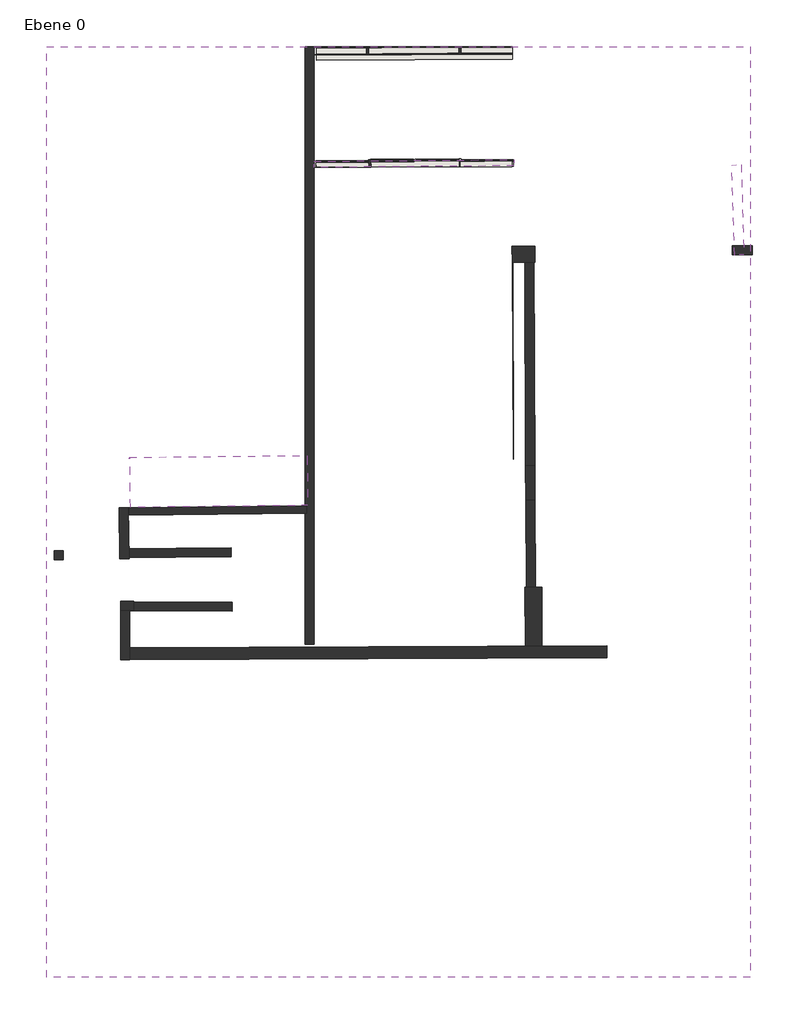
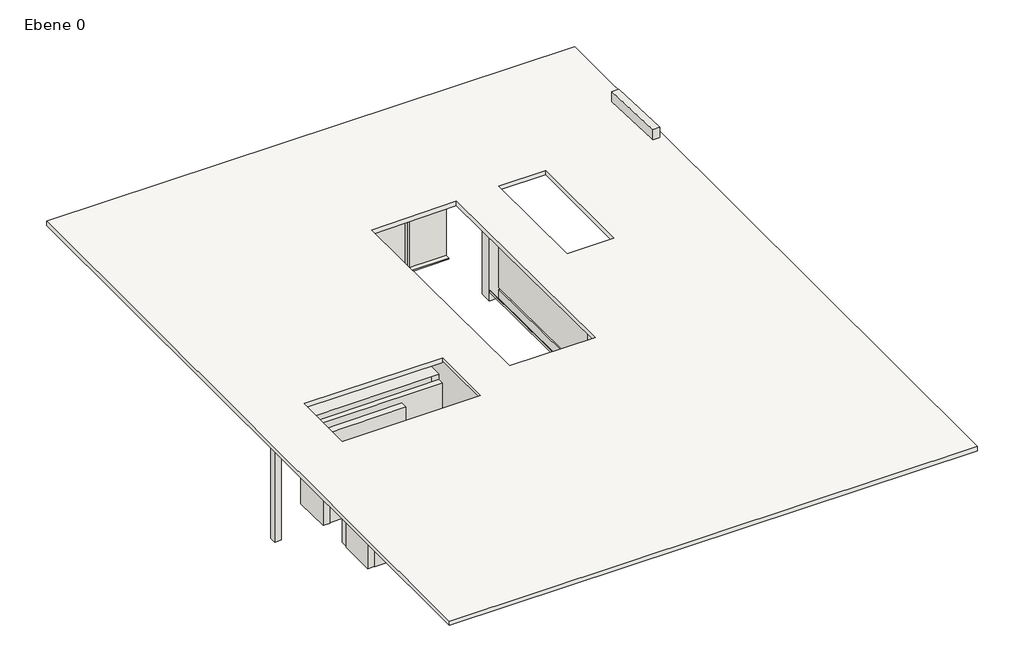
# One storey: 46 walls, 1 slab.
"""IFC4 building model written with IfcOpenShell, lengths in millimetres."""

from ifc_helpers import new_model, si_unit, frame, origin, place, context, project, spatial, polyline, outline, extrude, faceted_brep, element, save

model = new_model("IFC4")

# Units and contexts
model_context = context("Model", 3, world=origin())
ifc_project = project(units=[si_unit("LENGTHUNIT", "METRE", prefix="MILLI")], contexts=[model_context])

# Site, building, storey
site = spatial("IfcSite", under=ifc_project)
building = spatial("IfcBuilding", under=site)
storey = spatial("IfcBuildingStorey", under=building, Name="Ebene 0", Elevation=0.0)

# Slab
placement = place(None, origin())
element("IfcSlab", 1, ObjectType="STB 20.0", at=placement, inside=storey, context=model_context, shape_type="SweptSolid", body=[
    extrude(outline(polyline([(-11157.8712691, 14929.5123719), (12093.7927353, 14929.5123719), (12093.7927353, -15793.3401329), (-11157.8712691, -15793.3401329), (-11157.8712691, 14929.5123719)]), holes=[polyline([(-714.2464416, 8224.8662101), (-668.7269694, -2221.6847127), (3095.1356268, -2221.8899612), (3040.6752554, 8277.9612695), (-714.2464416, 8224.8662101)]), polyline([(4959.6247998, 8341.5505497), (4959.6247998, 3140.1225236), (7016.8801574, 3140.1225236), (7016.8801574, 8341.5505497), (4959.6247998, 8341.5505497)]), polyline([(-2623.9258692, -3380.2933626), (-2623.9258692, -499.2133132), (-8707.8712691, -499.2133132), (-8707.8712691, -3380.2933626), (-2623.9258692, -3380.2933626)])]), frame((0.0, 0.0, 3005.0), z_axis=(0.0, 0.0, 1.0), x_axis=(1.0, 0.0, 0.0)), (0.0, 0.0, 1.0), 200.0),
])

# Walls
element("IfcWall", 2, ObjectType="STB 30.0 - Sichtbeton 1", at=placement, inside=storey, context=model_context, shape_type="SweptSolid", body=[
    extrude(outline(polyline([(-8402.8984862, -3386.1116182), (-5023.0576004, -3407.986993), (-5024.9992525, -3707.9807096), (-8404.8401383, -3686.1053348), (-8402.8984862, -3386.1116182)])), frame((0.0, 0.0, -1567.0079424), z_axis=(0.0, 0.0, 1.0), x_axis=(1.0, 0.0, 0.0)), (0.0, 0.0, 1.0), 4193.9637451),
])
element("IfcWall", 3, ObjectType="STB 30.0 - Sichtbeton 1", at=placement, inside=storey, context=model_context, shape_type="SweptSolid", body=[
    extrude(outline(polyline([(-8711.881099, -1641.309095), (-5062.179794, -1608.676683), (-5059.4975656, -1908.6646922), (-8709.1988706, -1941.2971042), (-8711.881099, -1641.309095)])), frame((0.0, 0.0, -1566.6113359), z_axis=(0.0, 0.0, 1.0), x_axis=(1.0, 0.0, 0.0)), (0.0, 0.0, 1.0), 4193.494873),
])
element("IfcWall", 4, ObjectType="STB 30.0 - Sichtbeton 1", at=placement, inside=storey, context=model_context, shape_type="Brep", body=[
    faceted_brep([(-8280.7224922, -3375.8727385, -1505.4189133), (-8707.8712691, -3380.2933626, -1505.4189133), (-8707.8712691, -3380.2933626, 2636.550325), (-8280.7224922, -3375.8727385, 2636.550325), (-8280.7224922, -3375.8727385, -1388.9973215), (-8280.4523049, -3675.8860076, -1505.4189133), (-8280.4523049, -3675.8860076, 2636.550325), (-8407.8712691, -3677.2046848, 2636.550325), (-8707.8712691, -3680.3094278, 2636.550325), (-8707.8712691, -3680.3094278, -1505.4189133)], [[[0, 1, 2, 3, 4]], [[5, 6, 7, 8, 9]], [[1, 0, 5, 9]], [[3, 2, 8, 7, 6]], [[0, 4, 3, 6, 5]], [[2, 1, 9, 8]]]),
])
element("IfcWall", 5, ObjectType="STB 30.0 - Sichtbeton 1", at=placement, inside=storey, context=model_context, shape_type="Brep", body=[
    faceted_brep([(-8407.8712691, -5310.6242916, -1565.0), (-8407.8712691, -3677.2046848, -1565.0), (-8407.8712691, -3677.2046848, 2636.550325), (-8407.8712691, -5310.6242916, 2636.550325), (-8707.8712691, -5312.0476748, -1565.0), (-8707.8712691, -5312.0476748, 2636.550325), (-8707.8712691, -3680.3094278, 2636.550325), (-8707.8712691, -3680.3094278, -1505.4189133), (-8707.8712691, -3680.3094278, -1565.0)], [[[0, 1, 2, 3]], [[4, 5, 6, 7, 8]], [[1, 0, 4, 8]], [[3, 2, 6, 5]], [[2, 1, 8, 7, 6]], [[0, 3, 5, 4]]]),
])
element("IfcWall", 6, ObjectType="STB 30.0 - Sichtbeton 1", at=placement, inside=storey, context=model_context, shape_type="SweptSolid", body=[
    extrude(outline(polyline([(-8454.8872938, -283.8713377), (-8435.0535607, -1969.7388339), (-8735.0328016, -1973.268001), (-8754.8665347, -287.4005048), (-8454.8872938, -283.8713377)])), frame((0.0, 0.0, -1567.5369553), z_axis=(0.0, 0.0, 1.0), x_axis=(1.0, 0.0, 0.0)), (0.0, 0.0, 1.0), 4195.9727783),
])
element("IfcWall", 7, ObjectType="STB 30.0 - Sichtbeton 1", at=placement, inside=storey, context=model_context, shape_type="SweptSolid", body=[
    extrude(outline(polyline([(-10898.8481887, -2010.6735209), (-10902.7495019, -1710.7000992), (-10602.7748702, -1706.7987702), (-10598.873557, -2006.772192), (-10898.8481887, -2010.6735209)])), frame((0.0, 0.0, -1564.2386155), z_axis=(0.0, 0.0, 1.0), x_axis=(1.0, 0.0, 0.0)), (0.0, 0.0, 1.0), 4321.9161377),
])
element("IfcWall", 8, ObjectType="STB 30.0 - Sichtbeton 1", at=placement, inside=storey, context=model_context, shape_type="Brep", body=[
    faceted_brep([(4640.0905057, 7800.3536755, -1082.1717735), (4667.2831216, 1312.227188, -1082.1717735), (4667.2831216, 1312.227188, -1172.1717735), (4640.0905057, 7800.3536755, -1172.1717735), (4640.0905057, 7800.3536755, -1570.8115996), (4668.150891, 1105.1784267, -1570.8115996), (4668.150891, 1105.1784267, 3029.0079909), (4640.0905057, 7800.3536755, 3029.0079909), (4940.0878709, 7801.6110051, -1082.1717735), (4940.0878709, 7801.6110051, 3029.0079909), (4968.1456336, 1107.0614957, 3029.0079909), (4968.1456336, 1107.0614957, -1570.8115996), (4940.0878709, 7801.6110051, -1570.8115996), (4940.0878709, 7801.6110051, -1172.1717735), (4967.2804868, 1313.4845175, -1172.1717735), (4967.2804868, 1313.4845175, -1082.1717735)], [[[0, 1, 2, 3, 4, 5, 6, 7]], [[8, 9, 10, 11, 12, 13, 14, 15]], [[1, 0, 8, 15]], [[2, 1, 15, 14]], [[3, 2, 14, 13]], [[4, 3, 13, 12]], [[5, 4, 12, 11]], [[7, 6, 10, 9]], [[0, 7, 9, 8]], [[6, 5, 11, 10]]]),
])
element("IfcWall", 9, ObjectType="STB 30.0 - Sichtbeton 1", at=placement, inside=storey, context=model_context, shape_type="Brep", body=[
    faceted_brep([(4677.6567247, -31.4843616, 3026.055442), (4668.150891, 1105.1784267, 3026.055442), (4668.150891, 1105.1784267, 833.3), (4668.1769602, 1102.061196, 833.3), (4668.1769602, 1102.061196, 843.3), (4677.6567247, -31.4843616, 843.3), (4968.1456336, 1107.0614956, 3026.055442), (4977.6502256, -29.4528133, 3026.055442), (4977.6502256, -29.4528133, 843.3), (4968.1664699, 1104.5699879, 843.3), (4968.1664699, 1104.5699879, 833.3), (4968.1456336, 1107.0614956, 833.3)], [[[0, 1, 2, 3, 4, 5]], [[6, 7, 8, 9, 10, 11]], [[2, 11, 10, 3]], [[1, 0, 7, 6]], [[2, 1, 6, 11]], [[7, 0, 5, 8]], [[4, 9, 8, 5]], [[9, 4, 3, 10]]]),
])
element("IfcWall", 10, ObjectType="STB 30.0 - Sichtbeton 1", at=placement, inside=storey, context=model_context, shape_type="Brep", body=[
    faceted_brep([(4692.6152809, -2918.6509775, 3026.055442), (4677.6567247, -31.4843616, 3026.055442), (4677.6567247, -31.4843616, 843.3), (4677.6567247, -31.4843616, -1570.8115996), (4677.6744168, -34.8991368, -1570.8115996), (4692.6152809, -2918.6509775, -1570.8115996), (4992.6112545, -2917.0966832, 3026.055442), (4992.6112545, -2917.0966832, -1570.8115996), (4977.665445, -32.3903322, -1570.8115996), (4977.6502256, -29.4528134, -1570.8115996), (4977.6502256, -29.4528134, 843.3), (4977.6502256, -29.4528134, 3026.055442)], [[[0, 1, 2, 3, 4, 5]], [[6, 7, 8, 9, 10, 11]], [[1, 0, 6, 11]], [[5, 4, 3, 9, 8, 7]], [[0, 5, 7, 6]], [[3, 2, 1, 11, 10, 9]]]),
])
element("IfcWall", 11, ObjectType="STB 30.0 - Sichtbeton 1", at=placement, inside=storey, context=model_context, shape_type="Brep", body=[
    faceted_brep([(-2623.9258692, -4796.8405571, -1559.2743428), (-2623.9258692, -4796.8405571, 3034.8009859), (-2623.9258692, 14629.5579088, 3034.8009859), (-2623.9258692, 14919.5579088, 3034.8009859), (-2623.9258692, 14919.5579088, -1554.5282258), (-2623.9258692, 14939.5579088, -1554.5282258), (-2623.9258692, 14939.5579088, -1559.2743428), (-2623.9258692, 9821.2108055, -1559.2743428), (-2623.9258692, 9821.2108055, 843.3), (-2623.9258692, 8684.2108055, 843.3), (-2623.9258692, 8684.2108055, -1559.2743428), (-2623.9258692, 1234.2108055, -1559.2743428), (-2623.9258692, 1234.2108055, 843.3), (-2623.9258692, -25.7891945, 843.3), (-2623.9258692, -25.7891945, -1559.2743428), (-2323.9258692, -4796.8405571, 3034.8009859), (-2323.9258692, -4796.8405571, -1559.2743428), (-2323.9258692, -25.7891945, -1559.2743428), (-2323.9258692, -25.7891945, 843.3), (-2323.9258692, 1234.2108055, 843.3), (-2323.9258692, 1234.2108055, -1559.2743428), (-2323.9258692, 8684.2108055, -1559.2743428), (-2323.9258692, 8684.2108055, 843.3), (-2323.9258692, 9821.2108055, 843.3), (-2323.9258692, 9821.2108055, -1559.2743428), (-2323.9258692, 14939.5579088, -1559.2743428), (-2323.9258692, 14939.5579088, -1554.5282258), (-2323.9258692, 14919.5579088, -1554.5282258), (-2323.9258692, 14919.5579088, 3034.8009859), (-2473.9258692, 14919.5579088, 3034.8009859)], [[[0, 1, 2, 3, 4, 5, 6, 7, 8, 9, 10, 11, 12, 13, 14]], [[15, 16, 17, 18, 19, 20, 21, 22, 23, 24, 25, 26, 27, 28]], [[16, 0, 14, 17]], [[20, 11, 10, 21]], [[6, 25, 24, 7]], [[1, 0, 16, 15]], [[3, 2, 1, 15, 28, 29]], [[19, 12, 11, 20]], [[12, 19, 18, 13]], [[13, 18, 17, 14]], [[27, 26, 5, 4]], [[25, 6, 5, 26]], [[3, 29, 28, 27, 4]], [[23, 8, 7, 24]], [[8, 23, 22, 9]], [[9, 22, 21, 10]]]),
])
element("IfcWall", 12, ObjectType="STB 50.6 - Sichtbeton 9", at=placement, inside=storey, context=model_context, shape_type="Brep", body=[
    faceted_brep([(5199.7211413, -2916.1567546, 3026.055442), (5209.0004363, -4846.0130325, 3026.055442), (5209.0004363, -4846.0130325, -1564.9205192), (5199.7211413, -2916.1567546, -1571.9748716), (4649.727499, -2918.8012797, 3026.055442), (4649.727499, -2918.8012797, -1571.9748716), (4659.0066257, -4848.6225391, -1564.9206472), (4659.0066257, -4848.6225391, 3026.055442)], [[[0, 1, 2, 3]], [[4, 5, 6, 7]], [[1, 0, 4, 7]], [[3, 2, 6, 5]], [[0, 3, 5, 4]], [[2, 1, 7, 6]]]),
])
element("IfcWall", 13, ObjectType="STB 74.7 - Sichtbeton 8", at=placement, inside=storey, context=model_context, shape_type="SweptSolid", body=[
    extrude(outline(polyline([(4228.6457471, 7804.0053565), (4222.7195464, 8339.0935156), (4969.6737372, 8347.3661719), (4975.5999379, 7812.2780129), (4228.6457471, 7804.0053565)])), frame((0.0, 0.0, -1567.3220279), z_axis=(0.0, 0.0, 1.0), x_axis=(1.0, 0.0, 0.0)), (0.0, 0.0, 1.0), 4596.1280025),
])
element("IfcWall", 14, ObjectType="Sitzfläche Holz", at=placement, inside=storey, context=model_context, shape_type="SweptSolid", body=[
    extrude(outline(polyline([(4258.6670419, 1310.5146227), (4231.3829908, 7820.4574474), (4246.382859, 7820.5203138), (4273.6669102, 1310.5774892), (4258.6670419, 1310.5146227)])), frame((0.0, 0.0, -1172.1717735), z_axis=(0.0, 0.0, 1.0), x_axis=(1.0, 0.0, 0.0)), (0.0, 0.0, 1.0), 90.0),
])
element("IfcWall", 15, ObjectType="STB 30.0 - Sichtbeton 1", at=placement, inside=storey, context=model_context, shape_type="SweptSolid", body=[
    extrude(outline(polyline([(12156.2341991, 8065.3489209), (11495.6579868, 8063.6866533), (11494.9030721, 8363.6857035), (12156.2341991, 8365.3498707), (12156.2341991, 8065.3489209)])), frame((0.0, 0.0, -1554.8786442), z_axis=(0.0, 0.0, 1.0), x_axis=(1.0, 0.0, 0.0)), (0.0, 0.0, 1.0), 4605.4604069),
])
element("IfcWall", 16, ObjectType="STB 30.83 - Sichtbeton 10", at=placement, inside=storey, context=model_context, shape_type="SweptSolid", body=[
    extrude(outline(polyline([(11572.0416954, 8053.8502546), (11479.0551765, 11028.3975788), (11787.463897, 11029.737379), (11880.1911653, 8063.4832318), (11572.0416954, 8053.8502546)])), frame((0.0, 0.0, 3050.5817627), z_axis=(0.0, 0.0, 1.0), x_axis=(1.0, 0.0, 0.0)), (0.0, 0.0, 1.0), 634.2195252),
])
element("IfcWall", 17, ObjectType="Aluminiumrahmen 20cm", at=placement, inside=storey, context=model_context, shape_type="SweptSolid", body=[
    extrude(outline(polyline([(2530.9541861, 14704.8542909), (2466.9708915, 14706.1136197), (2470.9065593, 14906.0748922), (2534.889854, 14904.8155634), (2530.9541861, 14704.8542909)])), frame((0.0, 0.0, 963.2543258), z_axis=(0.0, 0.0, 1.0), x_axis=(1.0, 0.0, 0.0)), (0.0, 0.0, 1.0), 2077.8103027),
])
element("IfcWall", 18, ObjectType="Aluminiumrahmen 20cm", at=placement, inside=storey, context=model_context, shape_type="SweptSolid", body=[
    extrude(outline(polyline([(-516.6643868, 14688.191302), (-578.6088919, 14686.1559043), (-585.1770282, 14886.0480242), (-523.2325231, 14888.0834218), (-516.6643868, 14688.191302)])), frame((0.0, 0.0, 943.714653), z_axis=(0.0, 0.0, 1.0), x_axis=(1.0, 0.0, 0.0)), (0.0, 0.0, 1.0), 2096.5111084),
])
element("IfcWall", 19, ObjectType="Aluminiumrahmen 20cm", at=placement, inside=storey, context=model_context, shape_type="SweptSolid", body=[
    extrude(outline(polyline([(4241.1128382, 14525.186891), (-2240.5965186, 14482.3735992), (-2241.9175392, 14682.3692364), (4239.7918176, 14725.1825282), (4241.1128382, 14525.186891)])), frame((0.0, 0.0, 843.7151021), z_axis=(0.0, 0.0, 1.0), x_axis=(1.0, 0.0, 0.0)), (0.0, 0.0, 1.0), 99.9995509),
])
element("IfcWall", 20, ObjectType="Aluminiumrahmen 20cm", at=placement, inside=storey, context=model_context, shape_type="SweptSolid", body=[
    extrude(outline(polyline([(-454.8472123, 14616.4759781), (-496.8404301, 14616.0682776), (-498.7820831, 14816.0588524), (-456.7888653, 14816.4665529), (-454.8472123, 14616.4759781)])), frame((0.0, 0.0, -1569.2346878), z_axis=(0.0, 0.0, 1.0), x_axis=(1.0, 0.0, 0.0)), (0.0, 0.0, 1.0), 2407.9493408),
])
element("IfcWall", 21, ObjectType="Aluminiumrahmen 20cm", at=placement, inside=storey, context=model_context, shape_type="SweptSolid", body=[
    extrude(outline(polyline([(2451.6323777, 14636.0619156), (2403.6349929, 14636.4288193), (2405.163797, 14836.4229761), (2453.1611817, 14836.0560724), (2451.6323777, 14636.0619156)])), frame((0.0, 0.0, -1577.3386917), z_axis=(0.0, 0.0, 1.0), x_axis=(1.0, 0.0, 0.0)), (0.0, 0.0, 1.0), 2417.8755493),
])
element("IfcWall", 22, ObjectType="Aluminiumrahmen 20cm", at=placement, inside=storey, context=model_context, shape_type="SweptSolid", body=[
    extrude(outline(polyline([(-511.3662078, 10959.1183238), (-2319.8050257, 10959.1183238), (-2319.8050257, 11159.1183238), (-524.3930979, 11159.1183238), (-511.3662078, 10959.1183238)])), frame((0.0, 0.0, -1559.5502865), z_axis=(0.0, 0.0, 1.0), x_axis=(1.0, 0.0, 0.0)), (0.0, 0.0, 1.0), 51.7003161),
])
element("IfcWall", 23, ObjectType="Aluminiumrahmen 20cm 2", at=placement, inside=storey, context=model_context, shape_type="Brep", body=[
    faceted_brep([(-517.7933076, 11107.2777111, 900.0290089), (-517.9039135, 11105.9366786, 830.8928121), (-2250.633074, 11096.6298964, 833.8454007), (-2250.5224681, 11097.9709289, 902.9815975), (-2246.3874205, 11097.993139, 902.9745513), (-516.982536, 10957.2517121, 900.0290005), (-2245.5766498, 10947.96714, 902.9745429), (-2249.7116965, 10947.94493, 902.981589), (-2249.8223023, 10946.6038975, 833.8453923), (-517.0931419, 10955.9106796, 830.8928037)], [[[0, 1, 2, 3, 4]], [[5, 6, 7, 8, 9]], [[6, 5, 0, 4]], [[7, 6, 4, 3]], [[8, 7, 3, 2]], [[9, 8, 2, 1]], [[5, 9, 1, 0]]]),
])
element("IfcWall", 24, ObjectType="Aluminiumrahmen 20cm", at=placement, inside=storey, context=model_context, shape_type="SweptSolid", body=[
    extrude(outline(polyline([(2469.8899389, 10967.7043533), (-436.297192, 10960.4986908), (-449.3220187, 11160.4670115), (2469.3940561, 11167.7037385), (2469.8899389, 10967.7043533)])), frame((0.0, 0.0, 845.0347098), z_axis=(0.0, 0.0, 1.0), x_axis=(1.0, 0.0, 0.0)), (0.0, 0.0, 1.0), 43.8113839),
])
element("IfcWall", 25, ObjectType="Aluminiumrahmen 20cm", at=placement, inside=storey, context=model_context, shape_type="SweptSolid", body=[
    extrude(outline(polyline([(2532.2919931, 10975.5580245), (2470.5434806, 10975.7530127), (2471.1750336, 11175.7520156), (2532.9235461, 11175.5570273), (2532.2919931, 10975.5580245)])), frame((0.0, 0.0, -1500.4766489), z_axis=(0.0, 0.0, 1.0), x_axis=(1.0, 0.0, 0.0)), (0.0, 0.0, 1.0), 2345.5113587),
])
element("IfcWall", 26, ObjectType="Aluminiumrahmen 20cm", at=placement, inside=storey, context=model_context, shape_type="SweptSolid", body=[
    extrude(outline(polyline([(4289.3014273, 11005.4129185), (-2323.9258692, 10949.913032), (-2323.9258692, 11149.9200748), (4287.6230355, 11205.4058759), (4289.3014273, 11005.4129185)])), frame((0.0, 0.0, 2944.3505388), z_axis=(0.0, 0.0, 1.0), x_axis=(1.0, 0.0, 0.0)), (0.0, 0.0, 1.0), 86.6759664),
])
element("IfcWall", 27, ObjectType="Aluminiumrahmen 7,5cm", at=placement, inside=storey, context=model_context, shape_type="Brep", body=[
    faceted_brep([(-527.7117506, 11210.0691291, -1569.6072614), (-511.3662078, 10959.1183238, -1569.6072614), (-511.3662078, 10959.1183238, -1559.5502865), (-511.3662078, 10959.1183238, -1507.8499703), (-511.3662078, 10959.1183238, 2939.2424872), (-527.7117506, 11210.0691291, 2939.2424872), (-452.5886485, 11210.6191171, -1569.6072614), (-452.5886485, 11210.6191171, -1567.5099596), (-452.5886485, 11210.6191171, -1496.0611809), (-452.5886485, 11210.6191171, 2939.2424872), (-449.2570055, 11159.4688725, 2939.2424872), (-447.9543486, 11139.4693654, 2939.2424872), (-436.2072826, 10959.1183238, 2939.2424872), (-436.2072826, 10959.1183238, -1569.6072614)], [[[0, 1, 2, 3, 4, 5]], [[6, 7, 8, 9, 10, 11, 12, 13]], [[1, 0, 6, 13]], [[5, 4, 12, 11, 10, 9]], [[0, 5, 9, 8, 7, 6]], [[4, 3, 2, 1, 13, 12]]]),
])
element("IfcWall", 28, ObjectType="Aluminiumrahmen 20cm", at=placement, inside=storey, context=model_context, shape_type="SweptSolid", body=[
    extrude(outline(polyline([(4269.9303642, 10986.7075357), (2532.309784, 10981.1059862), (2531.6650494, 11181.104947), (4269.2856297, 11186.7064965), (4269.9303642, 10986.7075357)])), frame((0.0, 0.0, -1572.0237871), z_axis=(0.0, 0.0, 1.0), x_axis=(1.0, 0.0, 0.0)), (0.0, 0.0, 1.0), 62.3798925),
])
element("IfcWall", 29, ObjectType="Aluminiumrahmen 7,5cm", at=placement, inside=storey, context=model_context, shape_type="SweptSolid", body=[
    extrude(outline(polyline([(-452.5886485, 11210.6191171), (2478.4739757, 11232.0778854), (2479.0230477, 11157.0798953), (-447.7057623, 11135.6528555), (-452.5886485, 11210.6191171)])), frame((0.0, 0.0, -1567.5099596), z_axis=(0.0, 0.0, 1.0), x_axis=(1.0, 0.0, 0.0)), (0.0, 0.0, 1.0), 71.4487787),
])
element("IfcWall", 30, ObjectType="Aluminiumrahmen 20cm", at=placement, inside=storey, context=model_context, shape_type="SweptSolid", body=[
    extrude(outline(polyline([(2471.3474726, 11230.3596849), (2533.1410335, 11230.1645544), (2532.5094805, 11030.1655516), (2470.7159196, 11030.3606821), (2471.3474726, 11230.3596849)])), frame((0.0, 0.0, -1500.4766489), z_axis=(0.0, 0.0, 1.0), x_axis=(1.0, 0.0, 0.0)), (0.0, 0.0, 1.0), 2364.2643211),
])
element("IfcWall", 31, ObjectType="Aluminiumrahmen 20cm", at=placement, inside=storey, context=model_context, shape_type="SweptSolid", body=[
    extrude(outline(polyline([(4223.9186032, 10974.0579882), (2515.9054307, 10963.4053804), (2514.6580866, 11163.4014907), (4222.6712591, 11174.0540985), (4223.9186032, 10974.0579882)])), frame((0.0, 0.0, 845.0347098), z_axis=(0.0, 0.0, 1.0), x_axis=(1.0, 0.0, 0.0)), (0.0, 0.0, 1.0), 43.0983678),
])
element("IfcWall", 32, ObjectType="Aluminiumrahmen 20cm", at=placement, inside=storey, context=model_context, shape_type="SweptSolid", body=[
    extrude(outline(polyline([(-2243.2780557, 14888.3443346), (4238.4313012, 14931.1576264), (4239.7523218, 14731.1619892), (-2241.9570351, 14688.3486974), (-2243.2780557, 14888.3443346)])), frame((0.0, 0.0, 843.7151021), z_axis=(0.0, 0.0, 1.0), x_axis=(1.0, 0.0, 0.0)), (0.0, 0.0, 1.0), 99.9995509),
])
element("IfcWall", 33, ObjectType="Aluminiumrahmen 20cm", at=placement, inside=storey, context=model_context, shape_type="SweptSolid", body=[
    extrude(outline(polyline([(2405.7294156, 14910.4157336), (2453.7268003, 14910.0488299), (2452.1979963, 14710.0546731), (2404.2006116, 14710.4215768), (2405.7294156, 14910.4157336)])), frame((0.0, 0.0, -1577.3386917), z_axis=(0.0, 0.0, 1.0), x_axis=(1.0, 0.0, 0.0)), (0.0, 0.0, 1.0), 2417.8755493),
])
element("IfcWall", 34, ObjectType="Aluminiumrahmen 20cm", at=placement, inside=storey, context=model_context, shape_type="SweptSolid", body=[
    extrude(outline(polyline([(-499.4616302, 14886.0523207), (-457.4684125, 14886.4600212), (-455.5267595, 14686.4694465), (-497.5199772, 14686.0617459), (-499.4616302, 14886.0523207)])), frame((0.0, 0.0, -1569.2346878), z_axis=(0.0, 0.0, 1.0), x_axis=(1.0, 0.0, 0.0)), (0.0, 0.0, 1.0), 2407.9493408),
])
element("IfcWall", 35, ObjectType="Glasfassade", at=placement, inside=storey, context=model_context, shape_type="SweptSolid", body=[
    extrude(outline(polyline([(-449.2299687, 11212.4926831), (958.4892446, 11222.7988158), (958.6356638, 11202.7993518), (-449.0835495, 11192.4932191), (-449.2299687, 11212.4926831)])), frame((0.0, 0.0, -1496.0611809), z_axis=(0.0, 0.0, 1.0), x_axis=(1.0, 0.0, 0.0)), (0.0, 0.0, 1.0), 2344.345665),
])
element("IfcWall", 36, ObjectType="Glasfassade", at=placement, inside=storey, context=model_context, shape_type="SweptSolid", body=[
    extrude(outline(polyline([(1024.1639715, -19.9998824), (-1024.0267512, -19.9998823), (-1024.0953617, 0.0001177), (1024.095361, 0.0001177), (1024.1639715, -19.9998824)])), frame((-2241.2403215, 11125.2439305, 1920.2612034), z_axis=(0.9999647868922119, 0.00839195898543441, 0.0), x_axis=(-2.878865053450671e-05, 0.003430383399748157, 0.9999941158031603)), (0.0, 0.0, 1.0), 1723.3817094),
])
element("IfcWall", 37, ObjectType="Glasfassade", at=placement, inside=storey, context=model_context, shape_type="SweptSolid", body=[
    extrude(outline(polyline([(1028.3896086, -19.9987993), (-1027.9513066, -19.9987992), (-1028.1704708, 0.0012008), (1028.1704444, 0.0012008), (1028.3896086, -19.9987993)])), frame((2518.0878137, 11157.432084, 1916.2418082), z_axis=(0.999964786892212, 0.008391958985434413, 0.0), x_axis=(-9.195531599000662e-05, 0.010957164842832441, 0.9999399642392672)), (0.0, 0.0, 1.0), 1736.5032719),
])
element("IfcWall", 38, ObjectType="Glasfassade", at=placement, inside=storey, context=model_context, shape_type="SweptSolid", body=[
    extrude(outline(polyline([(4268.1486307, 11174.3377336), (2532.9787049, 11181.0998276), (2533.0566459, 11201.0996757), (4268.2265717, 11194.3375817), (4268.1486307, 11174.3377336)])), frame((0.0, 0.0, -1509.6438945), z_axis=(0.0, 0.0, 1.0), x_axis=(1.0, 0.0, 0.0)), (0.0, 0.0, 1.0), 2354.6786044),
])
element("IfcWall", 39, ObjectType="Glasfassade", at=placement, inside=storey, context=model_context, shape_type="SweptSolid", body=[
    extrude(outline(polyline([(-524.1136507, 11154.8280106), (-2249.5983951, 11147.9520531), (-2249.6780933, 11167.9518943), (-525.416012, 11174.8229795), (-524.1136507, 11154.8280106)])), frame((0.0, 0.0, -1507.8499703), z_axis=(0.0, 0.0, 1.0), x_axis=(1.0, 0.0, 0.0)), (0.0, 0.0, 1.0), 2334.8856416),
])
element("IfcWall", 40, ObjectType="Glasfassade", at=placement, inside=storey, context=model_context, shape_type="SweptSolid", body=[
    extrude(outline(polyline([(-449.2570055, 11159.4688725), (979.5144517, 11160.0111377), (979.5220423, 11140.0111392), (-447.9543486, 11139.4693654), (-449.2570055, 11159.4688725)])), frame((0.0, 0.0, 891.1173634), z_axis=(0.0, 0.0, 1.0), x_axis=(1.0, 0.0, 0.0)), (0.0, 0.0, 1.0), 2048.1251239),
])
element("IfcWall", 41, ObjectType="Glasfassade", at=placement, inside=storey, context=model_context, shape_type="SweptSolid", body=[
    extrude(outline(polyline([(1063.6949929, 11220.0540432), (2471.3474726, 11230.3596874), (2471.4938918, 11210.3602234), (1063.8414121, 11200.0545792), (1063.6949929, 11220.0540432)])), frame((0.0, 0.0, -1496.0611809), z_axis=(0.0, 0.0, 1.0), x_axis=(1.0, 0.0, 0.0)), (0.0, 0.0, 1.0), 2359.8488531),
])
element("IfcWall", 42, ObjectType="Glasfassade", at=placement, inside=storey, context=model_context, shape_type="SweptSolid", body=[
    extrude(outline(polyline([(1063.6949929, 11220.0540432), (2471.3474726, 11230.3596874), (2471.4938918, 11210.3602234), (1063.8414121, 11200.0545792), (1063.6949929, 11220.0540432)])), frame((0.0, 0.0, -1496.0611809), z_axis=(0.0, 0.0, 1.0), x_axis=(1.0, 0.0, 0.0)), (0.0, 0.0, 1.0), 2359.8488531),
])
element("IfcWall", 43, ObjectType="Glasfassade", at=placement, inside=storey, context=model_context, shape_type="Brep", body=[
    faceted_brep([(4235.0595919, 14919.5579088, -1554.5282258), (4235.0595919, 14919.5579088, 3035.7383094), (-2473.9258692, 14919.5579088, 3035.7383094), (-2473.9258692, 14919.5579088, 3034.8009859), (-2623.9258692, 14919.5579088, 3034.8009859), (-2623.9258692, 14919.5579088, -1554.5282258), (-2323.9258692, 14919.5579088, -1554.5282258), (4235.0595919, 14939.5579088, -1554.5282258), (-2323.9258692, 14939.5579088, -1554.5282258), (-2623.9258692, 14939.5579088, -1554.5282258), (-2623.9258692, 14939.5579088, 3034.8009859), (-2473.9258692, 14939.5579088, 3034.8009859), (-2473.9258692, 14939.5579088, 3035.7383094), (4235.0595919, 14939.5579088, 3035.7383094)], [[[0, 1, 2, 3, 4, 5, 6]], [[7, 8, 9, 10, 11, 12, 13]], [[1, 0, 7, 13]], [[2, 1, 13, 12]], [[0, 6, 5, 9, 8, 7]], [[3, 2, 12, 11]], [[3, 11, 10, 4]], [[5, 4, 10, 9]]]),
])
element("IfcWall", 44, ObjectType="Glasfassade", at=placement, inside=storey, context=model_context, shape_type="SweptSolid", body=[
    extrude(outline(polyline([(-2433.883637, 14669.1159954), (4236.984974, 14709.5666807), (4237.1062474, 14689.5670484), (-2433.7623637, 14649.116363), (-2433.883637, 14669.1159954)])), frame((0.0, 0.0, 894.7163796), z_axis=(0.0, 0.0, 1.0), x_axis=(1.0, 0.0, 0.0)), (0.0, 0.0, 1.0), 2140.7562727),
])
element("IfcWall", 45, ObjectType="STB 40.0 - Sichtbeton 7", at=placement, inside=storey, context=model_context, shape_type="Brep", body=[
    faceted_brep([(7358.7395645, -5235.8178592, -1577.6721536), (7358.7395645, -5235.8178592, 3028.7055287), (-8407.8712691, -5310.6242916, 3028.7055287), (-8407.8712691, -5310.6242916, 2636.550325), (-8407.8712691, -5310.6242916, -1565.0), (-8407.8712691, -5310.6242916, -1577.6721536), (-583.4447467, -5273.5004328, -1577.6721536), (-583.4447467, -5273.5004328, 843.3), (676.5410714, -5267.5222905, 843.3), (676.5410714, -5267.5222905, -1577.6721536), (726.8575404, -5267.2835584, -1577.6721536), (726.8575404, -5267.2835584, 843.3), (1986.8433585, -5261.3054161, 843.3), (1986.8433585, -5261.3054161, -1577.6721536), (7356.8417415, -4835.8223614, 3028.7055287), (7356.8417415, -4835.8223614, -1577.6721536), (1984.9455356, -4861.3099182, -1577.6721536), (1984.9455356, -4861.3099182, 843.3), (724.9597175, -4867.2880606, 843.3), (724.9597175, -4867.2880606, -1577.6721536), (674.6432484, -4867.5267927, -1577.6721536), (674.6432484, -4867.5267927, 843.3), (-585.3425697, -4873.504935, 843.3), (-585.3425697, -4873.504935, -1577.6721536), (-8407.8712691, -4910.6197893, -1577.6721536), (-8407.8712691, -4910.6197893, 3028.7055287)], [[[0, 1, 2, 3, 4, 5, 6, 7, 8, 9, 10, 11, 12, 13]], [[14, 15, 16, 17, 18, 19, 20, 21, 22, 23, 24, 25]], [[15, 0, 13, 16]], [[5, 24, 23, 6]], [[9, 20, 19, 10]], [[1, 0, 15, 14]], [[2, 1, 14, 25]], [[5, 4, 3, 2, 25, 24]], [[22, 7, 6, 23]], [[7, 22, 21, 8]], [[8, 21, 20, 9]], [[18, 11, 10, 19]], [[11, 18, 17, 12]], [[12, 17, 16, 13]]]),
])
element("IfcWall", 46, ObjectType="GK 25.0", at=placement, inside=storey, context=model_context, shape_type="SweptSolid", body=[
    extrude(outline(polyline([(0.0, 0.0), (3608.7078642, 0.0), (3608.6704113, -5888.6884598), (0.0266742, -5888.6884598), (0.0, 0.0)])), frame((-2563.8358921, -469.9186601, -1574.737862), z_axis=(-0.010857862877396351, 0.999941051669415, 0.0), x_axis=(0.0012161119308902936, 1.320515501101553e-05, 0.9999992604484242)), (0.0, 0.0, 1.0), 250.0),
])
element("IfcWall", 47, ObjectType="GK 25.0", at=placement, inside=storey, context=model_context, shape_type="SweptSolid", body=[
    extrude(outline(polyline([(-21540.6650721, 23920.4962764), (-26839.8897545, 21379.4135016), (-26859.1465615, 21419.6453465), (-27551.9062276, 22864.4135626), (-27174.8476023, 23045.1554225), (-22271.0517929, 25396.6222519), (-21577.9618072, 23952.0776279), (-21560.0463689, 23960.7073824), (-21540.6650721, 23920.4962764)])), frame((-17824.7416386, 32162.622769, 2048.895002), z_axis=(0.0012150993825128724, 0.00011277004424242195, 0.9999992554079268), x_axis=(-0.9061478884747843, 0.4229596844125457, 0.0010533633417530845)), (0.0, 0.0, 1.0), 250.0),
])

save(model, "model.ifc")

# Revit data of these elements
# Project information
#   Projektausgabedatum = "Projekt Datum"
#   Projektstatus = "Projektstatus"
#   Kundenname = "Bauherr"
#   Projektadresse = "Projektadresse"
#   Projektname = "Projektname"
#   Projektnummer = "Projektnummer"
#   Verfasser Firma 1 = "Firma 1"
#   Verfasser Firma 2 = "Firma 2"
#   Verfasser PLZ Ort = "PLZ Ort"
#   Verfasser Strasse = "Strasse"
#   Verfasser Telefon = "Telefon"
#   Verfasser Telefax = "Telefax"
#   Verfasser eMail = "E-Mail"
# Type "STB 20.0"
#   Function = 0
#   Layers, outside or top first: 0.200 m "Stahlbeton - Ortbeton" (function 1)
# Type "STB 30.0 - Sichtbeton 1"
#   Type Comments = "Stahlbeton Sichtbeton"
#   Description = "Stahlbeton (Sichtbeton) 30.0"
#   Layers, outside or top first: 0.300 m "Stahlbeton - Sichtbeton (1)" (function 1)
# Type "STB 50.6 - Sichtbeton 9"
#   Type Comments = "Stahlbeton Sichtbeton"
#   Description = "Stahlbeton (Sichtbeton) 30.0"
#   Layers, outside or top first: 0.550 m "Stahlbeton - Sichtbeton (1)" (function 1)
# Type "STB 74.7 - Sichtbeton 8"
#   Type Comments = "Stahlbeton Sichtbeton"
#   Description = "Stahlbeton (Sichtbeton) 30.0"
#   Layers, outside or top first: 0.747 m "Stahlbeton - Sichtbeton (1)" (function 1)
# Type "Sitzfläche Holz"
#   Type Comments = "Gipskarton"
#   Description = "1 x Gipskarton 1.25 cm, Metallständerprofil/Dämmung 7.5 cm, 1 x Gipskarton 1.25 cm"
#   Layers, outside or top first: 0.015 m "Holz - Birke" (function 2)
# Type "STB 30.83 - Sichtbeton 10"
#   Type Comments = "Stahlbeton Sichtbeton"
#   Description = "Stahlbeton (Sichtbeton) 30.0"
#   Layers, outside or top first: 0.3083 m "Stahlbeton - Sichtbeton (1)" (function 1)
# Type "Aluminiumrahmen 20cm"
#   Type Comments = "Standard"
#   Description = "Standardwand"
#   Layers, outside or top first: 0.200 m "Alumin." (function 1)
# Type "Aluminiumrahmen 20cm 2"
#   Type Comments = "Standard"
#   Description = "Standardwand"
#   Layers, outside or top first: 0.150 m "Alumin." (function 1)
# Type "Aluminiumrahmen 7,5cm"
#   Type Comments = "Standard"
#   Description = "Standardwand"
#   Layers, outside or top first: 0.075 m "Alumin." (function 1)
# Type "Glasfassade"
#   Type Comments = "Glasbaustein"
#   Description = "Glasbaustein 6.0 cm"
#   Layers, outside or top first: 0.020 m "Verglasung - Fensterverglasung" (function 1)
# Type "STB 40.0 - Sichtbeton 7"
#   Type Comments = "Stahlbeton Sichtbeton"
#   Description = "Stahlbeton (Sichtbeton) 30.0"
#   Layers, outside or top first: 0.400 m "Stahlbeton - Sichtbeton (1)" (function 1)
# Type "GK 25.0"
#   Type Comments = "Gipskarton"
#   Description = "2x Gipskarton 1.25 cm, Metallständerprofil/Dämmung 7.5 cm/ 5.0 cm/ 7.5 cm, 2x Gipskarton 1.25 cm"
#   Layers, outside or top first: 0.025 m "Gipswandbauplatte" (function 4); 0.075 m "Wärmedämmung - hart" (function 2); 0.050 m "Wärmedämmung - hart" (function 2); 0.075 m "Wärmedämmung - hart" (function 2); 0.025 m "Gipswandbauplatte" (function 5)
# Element 1 (IfcSlab, "STB 20.0")
#   built-in parameter 1001955 = 3.14159 (stored number, unit not read)
#   Height Offset From Level = 3.205 m
#   built-in parameter 1001954 = 1
#   Phase Created = Phase 1
#   Materials on its faces: "Stahlbeton - Ortbeton"
# Element 2 (IfcWall, "STB 30.0 - Sichtbeton 1")
#   built-in parameter 1001111 = -1.567008 m
#   Top Offset = 0.000 m
#   Base Offset = -1.567008 m
#   Unconnected Height = 4.193964 m
#   wall height = 4.193964 m
#   Phase Created = Phase 1
#   Base Constraint = Ebene 0
#   Materials on its faces: "Stahlbeton - Sichtbeton (1)"
# Element 3 (IfcWall, "STB 30.0 - Sichtbeton 1")
#   built-in parameter 1001111 = -1.566611 m
#   Top Offset = 0.000 m
#   Base Offset = -1.566611 m
#   Unconnected Height = 4.193495 m
#   wall height = 4.193495 m
#   Phase Created = Phase 1
#   Base Constraint = Ebene 0
#   Materials on its faces: "Stahlbeton - Sichtbeton (1)"
# Element 4 (IfcWall, "STB 30.0 - Sichtbeton 1")
#   built-in parameter 1001111 = -1.505419 m
#   Top Offset = 0.000 m
#   Base Offset = -1.505419 m
#   Unconnected Height = 4.141969 m
#   wall height = 4.141969 m
#   Phase Created = Phase 1
#   Base Constraint = Ebene 0
#   Materials on its faces: "Stahlbeton - Sichtbeton (1)"
# Element 5 (IfcWall, "STB 30.0 - Sichtbeton 1")
#   built-in parameter 1001111 = -1.565 m
#   Top Offset = 0.000 m
#   Base Offset = -1.565 m
#   Unconnected Height = 4.20155 m
#   wall height = 4.20155 m
#   Phase Created = Phase 1
#   Base Constraint = Ebene 0
#   Materials on its faces: "Stahlbeton - Sichtbeton (1)"
# Element 6 (IfcWall, "STB 30.0 - Sichtbeton 1")
#   built-in parameter 1001111 = -1.567537 m
#   Top Offset = 0.000 m
#   Base Offset = -1.567537 m
#   Unconnected Height = 4.195973 m
#   wall height = 4.195973 m
#   Phase Created = Phase 1
#   Base Constraint = Ebene 0
#   Materials on its faces: "Stahlbeton - Sichtbeton (1)"
# Element 7 (IfcWall, "STB 30.0 - Sichtbeton 1")
#   built-in parameter 1001111 = -1.564239 m
#   Top Offset = 0.000 m
#   Base Offset = -1.564239 m
#   Unconnected Height = 4.321916 m
#   wall height = 4.321916 m
#   Phase Created = Phase 1
#   Base Constraint = Ebene 0
#   Materials on its faces: "Stahlbeton - Sichtbeton (1)"
# Element 8 (IfcWall, "STB 30.0 - Sichtbeton 1")
#   built-in parameter 1001111 = -1.570812 m
#   Top Offset = 0.000 m
#   Base Offset = -1.570812 m
#   Unconnected Height = 4.59982 m
#   wall height = 4.59982 m
#   Phase Created = Phase 1
#   Base Constraint = Ebene 0
#   Materials on its faces: "Stahlbeton - Sichtbeton (1)"
# Element 9 (IfcWall, "STB 30.0 - Sichtbeton 1")
#   built-in parameter 1001111 = 0.8333 m
#   Top Offset = 0.000 m
#   Base Offset = 0.8333 m
#   Unconnected Height = 2.192755 m
#   wall height = 2.192755 m
#   Phase Created = Phase 1
#   Base Constraint = Ebene 0
#   Materials on its faces: "Stahlbeton - Sichtbeton (1)"
# Element 10 (IfcWall, "STB 30.0 - Sichtbeton 1")
#   built-in parameter 1001111 = -1.570812 m
#   Top Offset = 0.000 m
#   Base Offset = -1.570812 m
#   Unconnected Height = 4.596867 m
#   wall height = 4.596867 m
#   Phase Created = Phase 1
#   Base Constraint = Ebene 0
#   Materials on its faces: "Stahlbeton - Sichtbeton (1)"
# Element 11 (IfcWall, "STB 30.0 - Sichtbeton 1")
#   built-in parameter 1001111 = -1.559274 m
#   Top Offset = 0.000 m
#   Base Offset = -1.559274 m
#   Unconnected Height = 4.594075 m
#   wall height = 4.594075 m
#   Phase Created = Phase 1
#   Base Constraint = Ebene 0
#   Materials on its faces: "Stahlbeton - Sichtbeton (1)"
# Element 12 (IfcWall, "STB 50.6 - Sichtbeton 9")
#   built-in parameter 1001111 = -1.571975 m
#   Top Offset = 0.000 m
#   Base Offset = -1.571975 m
#   Unconnected Height = 4.59803 m
#   wall height = 4.59803 m
#   Phase Created = Phase 1
#   Base Constraint = Ebene 0
#   Materials on its faces: "Stahlbeton - Sichtbeton (1)"
# Element 13 (IfcWall, "STB 74.7 - Sichtbeton 8")
#   built-in parameter 1001111 = -1.567322 m
#   Top Offset = 0.000 m
#   Base Offset = -1.567322 m
#   Unconnected Height = 4.596128 m
#   wall height = 4.596128 m
#   Phase Created = Phase 1
#   Base Constraint = Ebene 0
#   Materials on its faces: "Stahlbeton - Sichtbeton (1)"
# Element 14 (IfcWall, "Sitzfläche Holz")
#   built-in parameter 1001111 = -1.172172 m
#   Top Offset = 0.000 m
#   Base Offset = -1.172172 m
#   Unconnected Height = 0.090 m
#   wall height = 0.090 m
#   Phase Created = Phase 1
#   Base Constraint = Ebene 0
#   Materials on its faces: "Holz - Birke"
# Element 15 (IfcWall, "STB 30.0 - Sichtbeton 1")
#   built-in parameter 1001111 = -1.554879 m
#   Top Offset = 0.000 m
#   Base Offset = -1.554879 m
#   Unconnected Height = 4.60546 m
#   wall height = 4.60546 m
#   Phase Created = Phase 1
#   Base Constraint = Ebene 0
#   Materials on its faces: "Stahlbeton - Sichtbeton (1)"
# Element 16 (IfcWall, "STB 30.83 - Sichtbeton 10")
#   built-in parameter 1001111 = 3.050582 m
#   Top Offset = 0.000 m
#   Base Offset = 3.050582 m
#   Unconnected Height = 0.63422 m
#   wall height = 0.63422 m
#   Phase Created = Phase 1
#   Base Constraint = Ebene 0
#   Materials on its faces: "Stahlbeton - Sichtbeton (1)"
# Element 17 (IfcWall, "Aluminiumrahmen 20cm")
#   built-in parameter 1001111 = 0.963254 m
#   Top Offset = 0.000 m
#   Base Offset = 0.963254 m
#   Unconnected Height = 2.07781 m
#   wall height = 2.07781 m
#   Phase Created = Phase 1
#   Base Constraint = Ebene 0
#   Materials on its faces: "Alumin."
# Element 18 (IfcWall, "Aluminiumrahmen 20cm")
#   built-in parameter 1001111 = 0.943715 m
#   Top Offset = 0.000 m
#   Base Offset = 0.943715 m
#   Unconnected Height = 2.096511 m
#   wall height = 2.096511 m
#   Phase Created = Phase 1
#   Base Constraint = Ebene 0
#   Materials on its faces: "Alumin."
# Elements 19, 32 (IfcWall, "Aluminiumrahmen 20cm")
#   built-in parameter 1001111 = 0.843715 m
#   Top Offset = 0.000 m
#   Base Offset = 0.843715 m
#   Unconnected Height = 0.100 m
#   wall height = 0.100 m
#   Phase Created = Phase 1
#   Base Constraint = Ebene 0
#   Materials on its faces: "Alumin."
# Elements 20, 34 (IfcWall, "Aluminiumrahmen 20cm")
#   built-in parameter 1001111 = -1.569235 m
#   Top Offset = 0.000 m
#   Base Offset = -1.569235 m
#   Unconnected Height = 2.407949 m
#   wall height = 2.407949 m
#   Phase Created = Phase 1
#   Base Constraint = Ebene 0
#   Materials on its faces: "Alumin."
# Elements 21, 33 (IfcWall, "Aluminiumrahmen 20cm")
#   built-in parameter 1001111 = -1.577339 m
#   Top Offset = 0.000 m
#   Base Offset = -1.577339 m
#   Unconnected Height = 2.417876 m
#   wall height = 2.417876 m
#   Phase Created = Phase 1
#   Base Constraint = Ebene 0
#   Materials on its faces: "Alumin."
# Element 22 (IfcWall, "Aluminiumrahmen 20cm")
#   built-in parameter 1001111 = -1.55955 m
#   Top Offset = 0.000 m
#   Base Offset = -1.55955 m
#   Unconnected Height = 0.0517 m
#   wall height = 0.0517 m
#   Phase Created = Phase 1
#   Base Constraint = Ebene 0
#   Materials on its faces: "Alumin."
# Element 23 (IfcWall, "Aluminiumrahmen 20cm 2")
#   Phase Created = Phase 1
#   Materials on its faces: "Alumin."
# Element 24 (IfcWall, "Aluminiumrahmen 20cm")
#   built-in parameter 1001111 = 0.845035 m
#   Top Offset = 0.000 m
#   Base Offset = 0.845035 m
#   Unconnected Height = 0.043811 m
#   wall height = 0.043811 m
#   Phase Created = Phase 1
#   Base Constraint = Ebene 0
#   Materials on its faces: "Alumin."
# Element 25 (IfcWall, "Aluminiumrahmen 20cm")
#   built-in parameter 1001111 = -1.500477 m
#   Top Offset = 0.000 m
#   Base Offset = -1.500477 m
#   Unconnected Height = 2.345511 m
#   wall height = 2.345511 m
#   Phase Created = Phase 1
#   Base Constraint = Ebene 0
#   Materials on its faces: "Alumin."
# Element 26 (IfcWall, "Aluminiumrahmen 20cm")
#   built-in parameter 1001111 = 2.944351 m
#   Top Offset = 0.000 m
#   Base Offset = 2.944351 m
#   Unconnected Height = 0.086676 m
#   wall height = 0.086676 m
#   Phase Created = Phase 1
#   Base Constraint = Ebene 0
#   Materials on its faces: "Alumin."
# Element 27 (IfcWall, "Aluminiumrahmen 7,5cm")
#   built-in parameter 1001111 = -1.569607 m
#   Top Offset = 0.000 m
#   Base Offset = -1.569607 m
#   Unconnected Height = 4.50885 m
#   wall height = 4.50885 m
#   Phase Created = Phase 1
#   Base Constraint = Ebene 0
#   Materials on its faces: "Alumin."
# Element 28 (IfcWall, "Aluminiumrahmen 20cm")
#   built-in parameter 1001111 = -1.572024 m
#   Top Offset = 0.000 m
#   Base Offset = -1.572024 m
#   Unconnected Height = 0.06238 m
#   wall height = 0.06238 m
#   Phase Created = Phase 1
#   Base Constraint = Ebene 0
#   Materials on its faces: "Alumin."
# Element 29 (IfcWall, "Aluminiumrahmen 7,5cm")
#   built-in parameter 1001111 = -1.56751 m
#   Top Offset = 0.000 m
#   Base Offset = -1.56751 m
#   Unconnected Height = 0.071449 m
#   wall height = 0.071449 m
#   Phase Created = Phase 1
#   Base Constraint = Ebene 0
#   Materials on its faces: "Alumin."
# Element 30 (IfcWall, "Aluminiumrahmen 20cm")
#   built-in parameter 1001111 = -1.500477 m
#   Top Offset = 0.000 m
#   Base Offset = -1.500477 m
#   Unconnected Height = 2.364264 m
#   wall height = 2.364264 m
#   Phase Created = Phase 1
#   Base Constraint = Ebene 0
#   Materials on its faces: "Alumin."
# Element 31 (IfcWall, "Aluminiumrahmen 20cm")
#   built-in parameter 1001111 = 0.845035 m
#   Top Offset = 0.000 m
#   Base Offset = 0.845035 m
#   Unconnected Height = 0.043098 m
#   wall height = 0.043098 m
#   Phase Created = Phase 1
#   Base Constraint = Ebene 0
#   Materials on its faces: "Alumin."
# Element 35 (IfcWall, "Glasfassade")
#   built-in parameter 1001111 = -1.496061 m
#   Top Offset = 0.000 m
#   Base Offset = -1.496061 m
#   Unconnected Height = 2.344346 m
#   wall height = 2.344346 m
#   Phase Created = Phase 1
#   Base Constraint = Ebene 0
#   Materials on its faces: "Verglasung - Fensterverglasung"
# Elements 36, 37 (IfcWall, "Glasfassade")
#   Phase Created = Phase 1
#   Materials on its faces: "Verglasung - Fensterverglasung"
# Element 38 (IfcWall, "Glasfassade")
#   built-in parameter 1001111 = -1.509644 m
#   Top Offset = 0.000 m
#   Base Offset = -1.509644 m
#   Unconnected Height = 2.354679 m
#   wall height = 2.354679 m
#   Phase Created = Phase 1
#   Base Constraint = Ebene 0
#   Materials on its faces: "Verglasung - Fensterverglasung"
# Element 39 (IfcWall, "Glasfassade")
#   built-in parameter 1001111 = -1.50785 m
#   Top Offset = 0.000 m
#   Base Offset = -1.50785 m
#   Unconnected Height = 2.334886 m
#   wall height = 2.334886 m
#   Phase Created = Phase 1
#   Base Constraint = Ebene 0
#   Materials on its faces: "Verglasung - Fensterverglasung"
# Element 40 (IfcWall, "Glasfassade")
#   built-in parameter 1001111 = 0.891117 m
#   Top Offset = 0.000 m
#   Base Offset = 0.891117 m
#   Unconnected Height = 2.048125 m
#   wall height = 2.048125 m
#   Phase Created = Phase 1
#   Base Constraint = Ebene 0
#   Materials on its faces: "Verglasung - Fensterverglasung"
# Elements 41, 42 (IfcWall, "Glasfassade")
#   built-in parameter 1001111 = -1.496061 m
#   Top Offset = 0.000 m
#   Base Offset = -1.496061 m
#   Unconnected Height = 2.359849 m
#   wall height = 2.359849 m
#   Phase Created = Phase 1
#   Base Constraint = Ebene 0
#   Materials on its faces: "Verglasung - Fensterverglasung"
# Element 43 (IfcWall, "Glasfassade")
#   built-in parameter 1001111 = -1.554528 m
#   Top Offset = 0.000 m
#   Base Offset = -1.554528 m
#   Unconnected Height = 4.590267 m
#   wall height = 4.590267 m
#   Phase Created = Phase 1
#   Base Constraint = Ebene 0
#   Materials on its faces: "Verglasung - Fensterverglasung", "Stahlbeton - Sichtbeton (1)"
# Element 44 (IfcWall, "Glasfassade")
#   built-in parameter 1001111 = 0.894716 m
#   Top Offset = 0.000 m
#   Base Offset = 0.894716 m
#   Unconnected Height = 2.140756 m
#   wall height = 2.140756 m
#   Phase Created = Phase 1
#   Base Constraint = Ebene 0
#   Materials on its faces: "Verglasung - Fensterverglasung"
# Element 45 (IfcWall, "STB 40.0 - Sichtbeton 7")
#   built-in parameter 1001111 = -1.577672 m
#   Top Offset = 0.000 m
#   Base Offset = -1.577672 m
#   Unconnected Height = 4.606378 m
#   wall height = 4.606378 m
#   Phase Created = Phase 1
#   Base Constraint = Ebene 0
#   Materials on its faces: "Stahlbeton - Sichtbeton (1)"
# Element 46 (IfcWall, "GK 25.0")
#   built-in parameter 1001111 = -1.575058 m
#   Top Offset = 0.000 m
#   Base Offset = -1.575058 m
#   Unconnected Height = 3.86614 m
#   wall height = 3.86614 m
#   Phase Created = Phase 1
#   Base Constraint = Ebene 0
#   Materials on its faces: "Gipswandbauplatte"
# Element 47 (IfcWall, "GK 25.0")
#   Phase Created = Phase 1
#   Materials on its faces: "Gipswandbauplatte"
# Materials
#   "Stahlbeton - Ortbeton": class "Beton", colour RGB 247 247 247, transparency 0, Cost = 0
#   "Stahlbeton - Sichtbeton (1)": class "Beton", colour RGB 192 192 192, transparency 0, Cost = 0
#   "Holz - Birke": class "Holz", colour RGB 213 164 103, transparency 0, Cost = 0
#   "Alumin.": class "Metall", colour RGB 247 247 247, transparency 0, Description = "Aluminium 6061", Cost = 0
#   "Verglasung - Fensterverglasung": class "Glas", colour RGB 0 128 192, transparency 0.75, Description = "Klarglas", Cost = 0
#   "Gipswandbauplatte": class "Allgemeines", colour RGB 228 228 228, transparency 0, Description = "Gipswandbauplatte", Cost = 0
#   "Wärmedämmung - hart": class "Stuck", colour RGB 255 255 255, transparency 0, Description = "Äußere Oberfläche", Cost = 0
